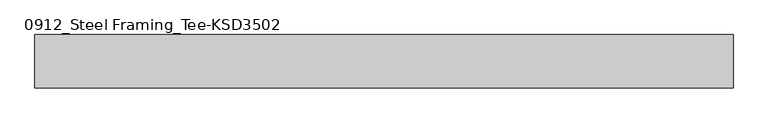
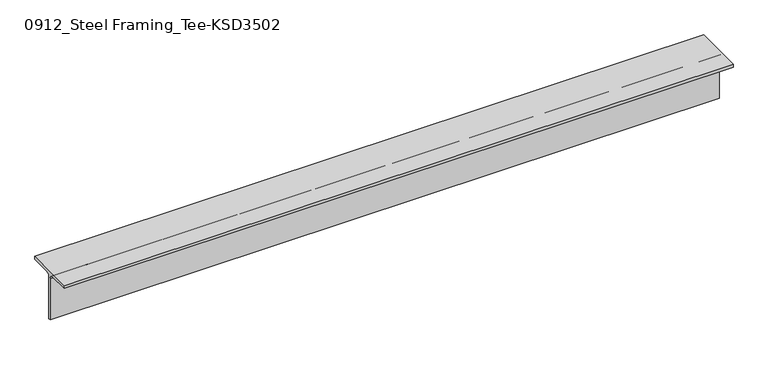
"""IFC4 building model written with IfcOpenShell, lengths in millimetres: member geometry, 0912_Steel Framing_Tee-KSD3502 : H_SB_ASB_CT-150x150x6.5x9."""

import ifcopenshell
import ifcopenshell.guid

model = None  # the IFC model being written
_history = None  # IfcOwnerHistory: only IFC2X3 demands one
_inside = {}  # id of a spatial element -> (the spatial element, [elements in it])
_under = {}  # id of a project, library or spatial element -> (it, [spatial elements below it])
_declared = {}  # id of a project -> (the project, [libraries it declares])
_typed = {}  # id of a type object -> (the type object, [elements of that type])
_made_of = {}  # id of a material, layer set ... -> (it, [elements and type objects made of it])


def new_model(schema):
    """Start an empty IFC model of exactly this schema.

    Asked for "IFC4X3", IfcOpenShell would pick the latest addendum, in which some entities
    have other attributes; the version numbers below select the first issue.
    IFC2X3 requires an IfcOwnerHistory on every rooted entity: one is made here for all.
    """
    global model, _history
    if schema == "IFC4X3":
        model = ifcopenshell.file(schema_version=(4, 3, 0, 0))
    else:
        model = ifcopenshell.file(schema=schema)
    _inside.clear()
    _under.clear()
    _declared.clear()
    _typed.clear()
    _made_of.clear()
    _history = None
    if model.schema == "IFC2X3":
        org = make("IfcOrganization", Name="unknown")
        user = make(
            "IfcPersonAndOrganization",
            ThePerson=make("IfcPerson", FamilyName="unknown"),
            TheOrganization=org,
        )
        app = make(
            "IfcApplication",
            ApplicationDeveloper=org,
            Version="unknown",
            ApplicationFullName="unknown",
            ApplicationIdentifier="unknown",
        )
        _history = make(
            "IfcOwnerHistory",
            OwningUser=user,
            OwningApplication=app,
            ChangeAction="ADDED",
            CreationDate=0,
        )
    return model


def make(cls, **values):
    """One entity of the class cls with the attributes given. An attribute that is None is left unset."""
    return model.create_entity(
        cls, **{name: value for name, value in values.items() if value is not None}
    )


def rooted(cls, **values):
    """An entity with a GlobalId (a new one), such as an element, a storey or a relation."""
    return make(cls, GlobalId=ifcopenshell.guid.new(), OwnerHistory=_history, **values)


def si_unit(unit_type, name, prefix=None):
    """IfcSIUnit, for example si_unit("LENGTHUNIT", "METRE", prefix="MILLI")."""
    return make("IfcSIUnit", UnitType=unit_type, Prefix=prefix, Name=name)


def assignment(units):
    """IfcUnitAssignment: the units of a project."""
    return None if units is None else make("IfcUnitAssignment", Units=units)


def point(xyz):
    """IfcCartesianPoint."""
    return None if xyz is None else make("IfcCartesianPoint", Coordinates=xyz)


def direction(xyz):
    """IfcDirection."""
    return None if xyz is None else make("IfcDirection", DirectionRatios=xyz)


def frame(location, z_axis=None, x_axis=None):
    """IfcAxis2Placement3D, a coordinate frame: its origin and axes. An axis left out is left unset."""
    return make(
        "IfcAxis2Placement3D",
        Location=point(location),
        Axis=direction(z_axis),
        RefDirection=direction(x_axis),
    )


def frame_2d(location, x_axis=None):
    """IfcAxis2Placement2D, a coordinate frame in the plane: its origin and x axis."""
    return make(
        "IfcAxis2Placement2D", Location=point(location), RefDirection=direction(x_axis)
    )


def origin():
    """The frame at (0, 0, 0) with its axes left unset."""
    return frame((0.0, 0.0, 0.0))


def place(relative_to, where):
    """IfcLocalPlacement: puts the frame where relative to a parent placement (None: the world)."""
    return make(
        "IfcLocalPlacement", PlacementRelTo=relative_to, RelativePlacement=where
    )


def context(
    kind, dimensions, precision=None, world=None, true_north=None, identifier=None
):
    """IfcGeometricRepresentationContext, for example the 3D "Model" context."""
    return make(
        "IfcGeometricRepresentationContext",
        ContextIdentifier=identifier,
        ContextType=kind,
        CoordinateSpaceDimension=dimensions,
        Precision=precision,
        WorldCoordinateSystem=world,
        TrueNorth=true_north,
    )


def project(units=None, contexts=None):
    """IfcProject with its units and contexts."""
    return rooted(
        "IfcProject",
        Name="project",
        RepresentationContexts=contexts,
        UnitsInContext=assignment(units),
    )


def spatial(cls, under=None, at=None, **own):
    """A site, building, storey or space (cls), placed at a placement, below another one or the project."""
    s = rooted(cls, ObjectPlacement=at, **own)
    if under is not None:
        _under.setdefault(under.id(), (under, []))[1].append(s)
    return s


def polyline(points):
    """IfcPolyline through the points."""
    return make("IfcPolyline", Points=[point(p) for p in points])


def circle_curve(where, radius):
    """IfcCircle in the frame where."""
    return make("IfcCircle", Position=where, Radius=radius)


def trimmed(basis, trim1, trim2, sense, master):
    """IfcTrimmedCurve: the piece of a basis curve between two trims."""
    return make(
        "IfcTrimmedCurve",
        BasisCurve=basis,
        Trim1=trim1,
        Trim2=trim2,
        SenseAgreement=sense,
        MasterRepresentation=master,
    )


def segment(curve, same_sense, transition):
    """IfcCompositeCurveSegment."""
    return make(
        "IfcCompositeCurveSegment",
        Transition=transition,
        SameSense=same_sense,
        ParentCurve=curve,
    )


def composite_curve(segments, self_intersect=None):
    """IfcCompositeCurve: segments joined end to end."""
    return make("IfcCompositeCurve", Segments=segments, SelfIntersect=self_intersect)


def outline(outer, holes=None, kind="AREA"):
    """IfcArbitraryClosedProfileDef: a profile drawn as a closed curve; with holes, ...WithVoids."""
    if holes is None:
        return make("IfcArbitraryClosedProfileDef", ProfileType=kind, OuterCurve=outer)
    return make(
        "IfcArbitraryProfileDefWithVoids",
        ProfileType=kind,
        OuterCurve=outer,
        InnerCurves=holes,
    )


def extrude(swept, where, along, depth):
    """IfcExtrudedAreaSolid: the profile swept, set in the frame where, extruded along a direction by depth."""
    return make(
        "IfcExtrudedAreaSolid",
        SweptArea=swept,
        Position=where,
        ExtrudedDirection=direction(along),
        Depth=depth,
    )


def shape(context_of_items, identifier, shape_type, items):
    """IfcShapeRepresentation: the items that make up one representation, for example the "Body"."""
    return make(
        "IfcShapeRepresentation",
        ContextOfItems=context_of_items,
        RepresentationIdentifier=identifier,
        RepresentationType=shape_type,
        Items=items,
    )


def source(mapping_origin, context_of_items, identifier, shape_type, items):
    """IfcRepresentationMap: a shape defined once, which mapped items show again and again."""
    return make(
        "IfcRepresentationMap",
        MappingOrigin=mapping_origin,
        MappedRepresentation=shape(context_of_items, identifier, shape_type, items),
    )


def transform(
    local_origin,
    x_axis=None,
    y_axis=None,
    z_axis=None,
    scale=None,
    scale2=None,
    scale3=None,
    uniform=True,
):
    """IfcCartesianTransformationOperator3D, or its non-uniform kind. x_axis, y_axis, z_axis: its Axis1, 2, 3."""
    if uniform:
        return make(
            "IfcCartesianTransformationOperator3D",
            Axis1=direction(x_axis),
            Axis2=direction(y_axis),
            LocalOrigin=point(local_origin),
            Scale=scale,
            Axis3=direction(z_axis),
        )
    return make(
        "IfcCartesianTransformationOperator3DnonUniform",
        Axis1=direction(x_axis),
        Axis2=direction(y_axis),
        LocalOrigin=point(local_origin),
        Scale=scale,
        Axis3=direction(z_axis),
        Scale2=scale2,
        Scale3=scale3,
    )


def mapped(mapping_source, mapping_target):
    """IfcMappedItem: shows the shape of a source again, moved by a transform."""
    return make(
        "IfcMappedItem", MappingSource=mapping_source, MappingTarget=mapping_target
    )


def made_of(thing, what):
    """Note that an element or type object is made of a material, layer set ...; save() writes the relation."""
    if what is not None:
        _made_of.setdefault(what.id(), (what, []))[1].append(thing)
    return thing


def element(
    cls,
    number,
    at=None,
    inside=None,
    cuts=None,
    type_object=None,
    material=None,
    context=None,
    identifier="Body",
    shape_type=None,
    held_by="IfcProductDefinitionShape",
    body=None,
    shapes=None,
    **own,
):
    """One element of the class cls, such as IfcWall. Its Tag is "e" and its number.

    at: its placement. inside: the storey or other place that contains it. cuts: it is an
    opening in that element (IfcRelVoidsElement). A single representation is given by context,
    identifier, shape_type and body (its items); several are given by shapes. held_by: the class
    of the entity that holds the representations. save() writes the other relations.
    """
    e = rooted(cls, Tag="e%d" % number, ObjectPlacement=at, **own)
    if body is not None:
        shapes = [shape(context, identifier, shape_type, body)]
    if shapes is not None:
        e.Representation = make(held_by, Representations=shapes)
    if inside is not None:
        _inside.setdefault(inside.id(), (inside, []))[1].append(e)
    if cuts is not None:
        rooted(
            "IfcRelVoidsElement", RelatingBuildingElement=cuts, RelatedOpeningElement=e
        )
    if type_object is not None:
        _typed.setdefault(type_object.id(), (type_object, []))[1].append(e)
    return made_of(e, material)


def aggregate(whole, parts):
    """IfcRelAggregates: a whole, such as a stair, and the parts it consists of."""
    return rooted("IfcRelAggregates", RelatingObject=whole, RelatedObjects=parts)


def save(model, path):
    """Write the relations noted so far, then the file.

    IfcRelAggregates (storeys below a building ...), IfcRelContainedInSpatialStructure (elements
    in a storey), IfcRelDefinesByType, IfcRelAssociatesMaterial and IfcRelDeclares: one each for
    every whole, place, type object, material and project.
    """
    for whole, parts in _under.values():
        aggregate(whole, parts)
    for where, things in _inside.values():
        rooted(
            "IfcRelContainedInSpatialStructure",
            RelatedElements=things,
            RelatingStructure=where,
        )
    for kind, things in _typed.values():
        rooted("IfcRelDefinesByType", RelatedObjects=things, RelatingType=kind)
    for what, things in _made_of.values():
        rooted("IfcRelAssociatesMaterial", RelatedObjects=things, RelatingMaterial=what)
    for by, libraries in _declared.values():
        rooted("IfcRelDeclares", RelatingContext=by, RelatedDefinitions=libraries)
    model.write(path)


def member_0912_steel_framing_tee_ksd3502_64e65919(model_context):
    return source(origin(), model_context, "Body", "SweptSolid", [
        extrude(outline(composite_curve([segment(polyline([(75.0, 75.0), (75.0, 66.0), (16.25, 66.0)]), True, "CONTINUOUS"), segment(trimmed(circle_curve(frame_2d((16.25, 53.0)), 13.0), [point((16.25, 66.0))], [point((3.25, 53.0))], True, "CARTESIAN"), True, "CONTINUOUS"), segment(polyline([(3.25, 53.0), (3.25, -75.0), (-3.25, -75.0), (-3.25, 53.0)]), True, "CONTINUOUS"), segment(trimmed(circle_curve(frame_2d((-16.25, 53.0)), 13.0), [point((-3.25, 53.0))], [point((-16.25, 66.0))], True, "CARTESIAN"), True, "CONTINUOUS"), segment(polyline([(-16.25, 66.0), (-75.0, 66.0), (-75.0, 75.0), (75.0, 75.0)]), True, "CONTINUOUS")], self_intersect=False)), frame((-983.95, 0.0, 0.0), z_axis=(1.0, 0.0, 0.0), x_axis=(0.0, 1.0, 0.0)), (0.0, 0.0, 1.0), 1967.9),
    ])


if __name__ == "__main__":
    model = new_model("IFC4")
    model_context = context("Model", 3, world=origin())
    ifc_project = project(units=[si_unit("LENGTHUNIT", "METRE", prefix="MILLI")], contexts=[model_context])
    site = spatial("IfcSite", under=ifc_project)
    building = spatial("IfcBuilding", under=site)
    placement = place(None, origin())
    member_0912_steel_framing_tee_ksd3502_shape = member_0912_steel_framing_tee_ksd3502_64e65919(model_context)
    element("IfcMember", 1, ObjectType="0912_Steel Framing_Tee-KSD3502 : H_SB_ASB_CT-150x150x6.5x9", at=placement, inside=building, context=model_context, shape_type="MappedRepresentation", body=[
        mapped(member_0912_steel_framing_tee_ksd3502_shape, transform((0.0, 0.0, 0.0), x_axis=(1.0, 0.0, 0.0), y_axis=(0.0, 1.0, 0.0), z_axis=(0.0, 0.0, 1.0))),
    ])
    save(model, "model.ifc")

# Revit data of these elements
# Type "0912_Steel Framing_Tee-KSD3502 : H_SB_ASB_CT-150x150x6.5x9"
#   H_WM Code_1 = "S01AA003-00001 | Main Steel Structure Fabrication Work | Shelter/Building | Light Steel - Standard (30KG/M>Weight) | Material: (   )"
#   H_WM Code_2 = "S03AA029-00001 | Main Steel Structure Erection Work | Shelter/Building | Light Steel (30KG/M>Weight) | Material: (   )"
#   H_WM Code_3 = "S01AA010-00001 | Main Steel Structure Fabrication Work | Shelter/Building | Steel Painting/Coating | for Non-Fireproofed Steel Surface, Surface Preparation, Primer, Second & Final Coat | Material: (   )"
#   H_Q'ty Cal Type Tag = "SB-Q2"
#   Width = 15.0 cm
#   Web Thickness = 0.65 cm
#   Web Fillet = 1.3 cm
#   Section Area = 23.39 cm²
#   Perimeter = 0.60 m²/m
#   Nominal Weight = 18.40 kgf/m
#   Height = 15.0 cm
#   Flange Thickness = 0.9 cm
#   Centroid Vertical = 7.5 cm
#   Centroid Horizontal = 7.5 cm
#   Length [instance default] = 1.5000 m
#   Structural Material [instance default] = Steel, 45-345
#   Warping Constant = (empty or 0)
#   Torsional Moment of Inertia = 0
#   Section Name Key = ""
#   Plastic Modulus weak axis = 0
#   Plastic Modulus strong axis = 0
#   Moment of Inertia weak axis = 0
#   Moment of Inertia strong axis = 0
#   Elastic Modulus weak axis = 0
#   Elastic Modulus strong axis = 0
#   Bolt Spacing = 0
#   Assembly Code = ""
# Element 1 (IfcMember, "0912_Steel Framing_Tee-KSD3502 : H_SB_ASB_CT-150x150x6.5x9")
#   Structural Material = none
# Materials
#   "Steel, 45-345": class "Metal", colour RGB 189 187 185, transparency 0, Description = "Steel 345 MPa", Cost = 0
